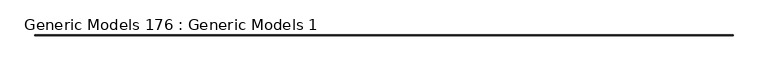
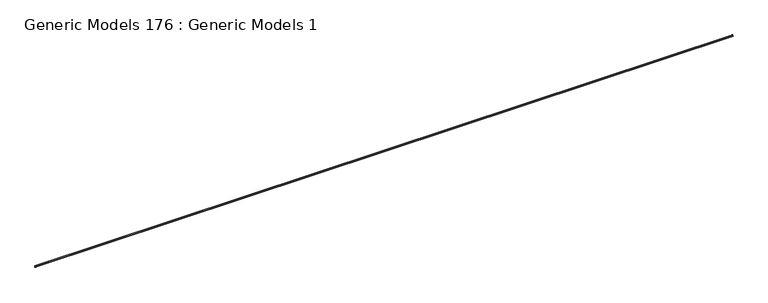
"""IFC4 building model written with IfcOpenShell, lengths in millimetres: proxy geometry, Generic Models 176 : Generic Models 1."""

from ifc_helpers import new_model, si_unit, frame, origin, place, context, project, spatial, polyline, outline, extrude, source, transform, mapped, element, save


def generic_models_176_generic_models_1_ab038d0e(model_context):
    return source(origin(), model_context, "Body", "SweptSolid", [
        extrude(outline(polyline([(-5471.9680827, 126847.3261596), (-5471.9680827, 126807.9561596), (-5473.2380827, 126807.9561596), (-5473.2380827, 126827.0061596), (-5492.9230827, 126827.0061596), (-5492.9230827, 126823.5263596), (-5494.1930827, 126823.5263596), (-5494.1930827, 126828.2761596), (-5473.2380827, 126828.2761596), (-5473.2380827, 126847.3261596), (-5471.9680827, 126847.3261596)])), frame((-16853.0736296, 0.0, 0.0), z_axis=(1.0, 0.0, 0.0), x_axis=(0.0, 1.0, 0.0)), (0.0, 0.0, 1.0), 19050.0),
    ])


if __name__ == "__main__":
    model = new_model("IFC4")
    model_context = context("Model", 3, world=origin())
    ifc_project = project(units=[si_unit("LENGTHUNIT", "METRE", prefix="MILLI")], contexts=[model_context])
    site = spatial("IfcSite", under=ifc_project)
    building = spatial("IfcBuilding", under=site)
    placement = place(None, origin())
    generic_models_176_generic_models_1_shape = generic_models_176_generic_models_1_ab038d0e(model_context)
    element("IfcBuildingElementProxy", 1, Name="Generic Models 176 : Generic Models 1", ObjectType="Generic Models 176 : Generic Models 1", at=placement, inside=building, context=model_context, shape_type="MappedRepresentation", body=[
        mapped(generic_models_176_generic_models_1_shape, transform((0.0, 0.0, 0.0), x_axis=(1.0, 0.0, 0.0), y_axis=(0.0, 1.0, 0.0), z_axis=(0.0, 0.0, 1.0))),
    ])
    save(model, "model.ifc")

# Revit data of these elements
# Element 1 (IfcBuildingElementProxy, "Generic Models 176 : Generic Models 1")
#   Materials on its faces: "_ 16 GA. COPPER VENTED T REVEAL BEAD"
# Materials
#   "_ 16 GA. COPPER VENTED T REVEAL BEAD": class "Generic", colour RGB 253 192 103, transparency 0, Cost = 0
